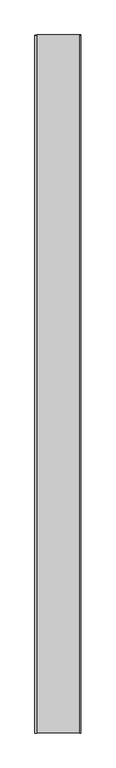
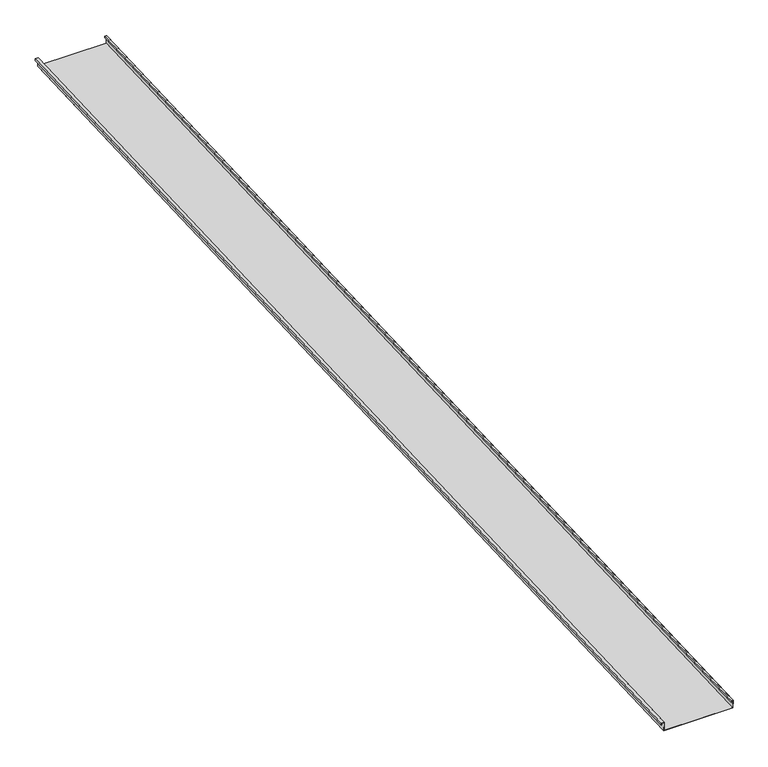
"""IFC4 building model written with IfcOpenShell, lengths in millimetres: proxy geometry, Generic Models 2:Generic Models 2:310765:Generic Models 2:310765 : Generic Models 2:Generic Models 2:310765:108 : Generic Models 2:Generic Models 2:310765:Generic Models 2:310765 : Generic Models 2:Generic Models 2:310765:300385."""

from ifc_helpers import new_model, si_unit, frame, origin, place, context, project, spatial, polyline, outline, extrude, source, transform, mapped, element, save


def generic_models_a621200c(model_context):
    return source(origin(), model_context, "Body", "SweptSolid", [
        extrude(outline(polyline([(1.5875, 0.0), (1.5875, 50.8), (407.9875, 50.8), (407.9875, 1.5875), (396.875, 1.5875), (396.875, 11.1125), (398.4625, 11.1125), (398.4625, 3.175), (406.4, 3.175), (406.4, 49.2125), (3.175, 49.2125), (3.175, -1.5874999), (-14.2875, -1.5874999), (-14.2875, 9.525), (-12.7, 9.525), (-12.7, 0.0), (1.5875, 0.0)])), frame((610693.9096406, -581354.4345603, 3902.6697972), z_axis=(0.0, 0.9991330730923568, 0.041630544712067834), x_axis=(1.0, 0.0, 0.0)), (0.0, 0.0, 1.0), 6400.8),
    ])


if __name__ == "__main__":
    model = new_model("IFC4")
    model_context = context("Model", 3, world=origin())
    ifc_project = project(units=[si_unit("LENGTHUNIT", "METRE", prefix="MILLI")], contexts=[model_context])
    site = spatial("IfcSite", under=ifc_project)
    building = spatial("IfcBuilding", under=site)
    placement = place(None, origin())
    generic_models_shape = generic_models_a621200c(model_context)
    element("IfcBuildingElementProxy", 1, Name="Generic Models 2:Generic Models 2:310765:Generic Models 2:310765 : Generic Models 2:Generic Models 2:310765:108 : Generic Models 2:Generic Models 2:310765:Generic Models 2:310765 : Generic Models 2:Generic Models 2:310765:300385", ObjectType="Generic Models 2:Generic Models 2:310765:Generic Models 2:310765 : Generic Models 2:Generic Models 2:310765:108 : Generic Models 2:Generic Models 2:310765:Generic Models 2:310765 : Generic Models 2:Generic Models 2:310765:300385", at=placement, inside=building, context=model_context, shape_type="MappedRepresentation", body=[
        mapped(generic_models_shape, transform((0.0, 0.0, 0.0), x_axis=(1.0, 0.0, 0.0), y_axis=(0.0, 1.0, 0.0), z_axis=(0.0, 0.0, 1.0))),
    ])
    save(model, "model.ifc")

# Revit data of these elements
# Type "Generic Models 2:Generic Models 2:310765:Generic Models 2:310765 : Generic Models 2:Generic Models 2:310765:108 : Generic Models 2:Generic Models 2:310765:Generic Models 2:310765 : Generic Models 2:Generic Models 2:310765:300385"
#   NameOverride = "Generic Models 2:Generic Models 2:310765:Generic Models 2:310765 : Generic Models 2:Generic Models 2:310765:300385"
#   ObjectTypeOverride = "Generic Models 2:310765 : Generic Models 2:Generic Models 2:310765"
#   Reference = "Generic Models 2"
#   Tag = "300385"
# Element 1 (IfcBuildingElementProxy, "Generic Models 2:Generic Models 2:310765:Generic Models 2:310765 : Generic Models 2:Generic Models 2:310765:108 : Generic Models 2:Generic Models 2:310765:Generic Models 2:310765 : Generic Models 2:Generic Models 2:310765:300385")
#   Materials on its faces: "THERMAL BROKEN ALUMINUM STOREFRONT FOR POLYCARBONATE"
# Materials
#   "THERMAL BROKEN ALUMINUM STOREFRONT FOR POLYCARBONATE": class "Unassigned", colour RGB 244 244 244, transparency 0, Keynote = "M07611300.01", Cost = 0
